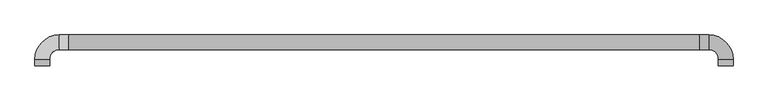
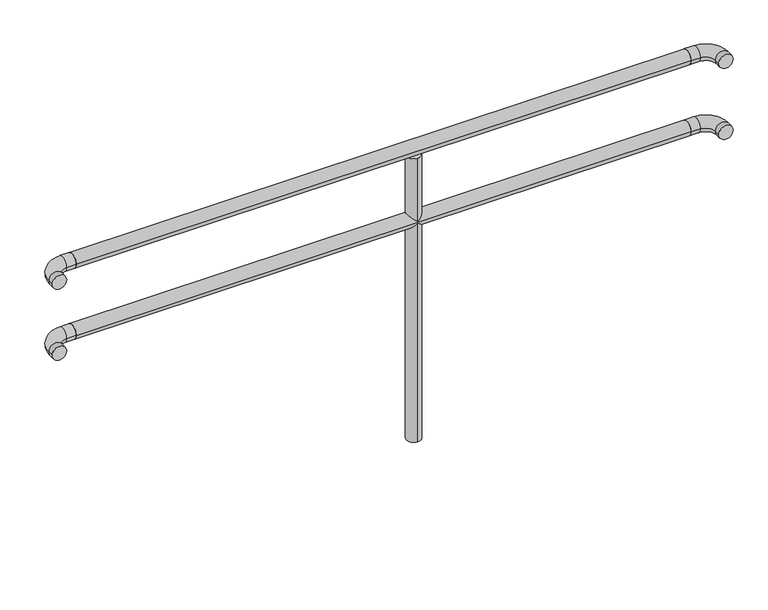
"""IFC4 building model written with IfcOpenShell, lengths in millimetres: railing geometry."""

from ifc_helpers import new_model, si_unit, point, frame, frame_2d, origin, origin_with_axes, place, context, project, spatial, circle_curve, ellipse_curve, trimmed, segment, composite_curve, outline, extrude, source, transform, mapped, element, save
from ifc_brep_helpers import plane_surface, cylinder_surface, revolved_surface, advanced_brep


def railing_ab6729c0(model_context):
    return source(origin(), model_context, "Body", "SolidModel", [
        extrude(outline(composite_curve([segment(trimmed(circle_curve(frame_2d((31458.1400611, 899.0)), 21.0), [point((31479.1400611, 899.0))], [point((31437.1400611, 899.0))], False, "CARTESIAN"), True, "CONTINUOUS"), segment(trimmed(circle_curve(frame_2d((31458.1400611, 899.0)), 21.0), [point((31437.1400611, 899.0))], [point((31479.1400611, 899.0))], False, "CARTESIAN"), True, "CONTINUOUS")], self_intersect=False)), frame((9766.6129185, 0.0, 0.0), z_axis=(1.0, 0.0, 0.0), x_axis=(0.0, 1.0, 0.0)), (0.0, 0.0, 1.0), 1800.0),
        extrude(outline(composite_curve([segment(trimmed(circle_curve(frame_2d((31458.1400611, 679.0)), 21.0), [point((31479.1400611, 679.0))], [point((31437.1400611, 679.0))], False, "CARTESIAN"), True, "CONTINUOUS"), segment(trimmed(circle_curve(frame_2d((31458.1400611, 679.0)), 21.0), [point((31437.1400611, 679.0))], [point((31479.1400611, 679.0))], False, "CARTESIAN"), True, "CONTINUOUS")], self_intersect=False)), frame((9766.6129185, 0.0, 0.0), z_axis=(1.0, 0.0, 0.0), x_axis=(0.0, 1.0, 0.0)), (0.0, 0.0, 1.0), 1800.0),
        extrude(outline(composite_curve([segment(trimmed(circle_curve(frame_2d((10766.6129185, 31458.1400611)), 21.0), [point((10766.6129185, 31479.1400611))], [point((10766.6129185, 31437.1400611))], False, "CARTESIAN"), True, "CONTINUOUS"), segment(trimmed(circle_curve(frame_2d((10766.6129185, 31458.1400611)), 21.0), [point((10766.6129185, 31437.1400611))], [point((10766.6129185, 31479.1400611))], False, "CARTESIAN"), True, "CONTINUOUS")], self_intersect=False)), origin_with_axes(), (0.0, 0.0, 1.0), 878.0),
        advanced_brep(
        [(11566.6129185, 31437.1900611, 679.1), (11566.6129185, 31479.1900611, 679.1), (11594.1129185, 31437.1900611, 679.1), (11594.1129185, 31479.1900611, 679.1), (11663.6129185, 31409.6900611, 679.1), (11621.6129185, 31409.6900611, 679.1), (11621.6129185, 31391.1900611, 679.1), (11663.6129185, 31391.1900611, 679.1)],
        [
            (0, 1, circle_curve(frame((11566.6129185, 31458.1900611, 679.1), z_axis=(-1.0, 0.0, 0.0), x_axis=(0.0, 1.0, 0.0)), 21.0)),
            (1, 0, circle_curve(frame((11566.6129185, 31458.1900611, 679.1), z_axis=(-1.0, 0.0, 0.0), x_axis=(0.0, 1.0, 0.0)), 21.0)),
            (0, 2),
            (2, 3, circle_curve(frame((11594.1129185, 31458.1900611, 679.1), z_axis=(-1.0, 0.0, 0.0), x_axis=(0.0, 1.0, 0.0)), 21.0)),
            (3, 1),
            (3, 2, circle_curve(frame((11594.1129185, 31458.1900611, 679.1), z_axis=(-1.0, 0.0, 0.0), x_axis=(0.0, 1.0, 0.0)), 21.0)),
            (4, 3, circle_curve(frame((11594.1129185, 31409.6900611, 679.1), z_axis=(0.0, 0.0, 1.0), x_axis=(0.0, 1.0, 0.0)), 69.5)),
            (2, 5, circle_curve(frame((11594.1129185, 31409.6900611, 679.1), z_axis=(0.0, 0.0, -1.0), x_axis=(0.0, 1.0, 0.0)), 27.5)),
            (5, 4, circle_curve(frame((11642.6129185, 31409.6900611, 679.1), z_axis=(0.0, 1.0, 0.0), x_axis=(1.0, 0.0, 0.0)), 21.0)),
            (4, 5, circle_curve(frame((11642.6129185, 31409.6900611, 679.1), z_axis=(0.0, 1.0, 0.0), x_axis=(1.0, 0.0, 0.0)), 21.0)),
            (6, 7, circle_curve(frame((11642.6129185, 31391.1900611, 679.1), z_axis=(0.0, -1.0, 0.0), x_axis=(1.0, 0.0, 0.0)), 21.0)),
            (7, 6, circle_curve(frame((11642.6129185, 31391.1900611, 679.1), z_axis=(0.0, -1.0, 0.0), x_axis=(1.0, 0.0, 0.0)), 21.0)),
            (5, 6),
            (7, 4),
        ],
        [
            plane_surface(frame((11566.6129185, 31458.1900611, 679.1), z_axis=(-1.0, 0.0, 0.0), x_axis=(0.0, 0.0, 1.0))),
            cylinder_surface(frame((11566.6129185, 31458.1900611, 679.1), z_axis=(-1.0, 0.0, 0.0), x_axis=(0.0, 1.0, 0.0)), 21.0),
            revolved_surface(trimmed(ellipse_curve(frame((11594.1129185, 31458.1900611, 679.1), z_axis=(-1.0, 0.0, 0.0), x_axis=(0.0, 1.0, 0.0)), 21.0, 21.0), [point((11594.1129185, 31437.1900611, 679.1))], [point((11594.1129185, 31479.1900611, 679.1))], True, "CARTESIAN"), (11594.1129185, 31409.6900611, 679.1), (0.0, 0.0, -1.0)),
            revolved_surface(trimmed(ellipse_curve(frame((11594.1129185, 31458.1900611, 679.1), z_axis=(-1.0, 0.0, 0.0), x_axis=(0.0, 1.0, 0.0)), 21.0, 21.0), [point((11594.1129185, 31479.1900611, 679.1))], [point((11594.1129185, 31437.1900611, 679.1))], True, "CARTESIAN"), (11594.1129185, 31409.6900611, 679.1), (0.0, 0.0, -1.0)),
            plane_surface(frame((11642.6129185, 31391.1900611, 679.1), z_axis=(0.0, -1.0, 0.0), x_axis=(0.0, 0.0, 1.0))),
            cylinder_surface(frame((11642.6129185, 31409.6900611, 679.1), z_axis=(0.0, 1.0, 0.0), x_axis=(1.0, 0.0, 0.0)), 21.0),
        ],
        [
            (0, [[1, 2]]),
            (1, [[-1, 3, 4, 5]]),
            (1, [[-2, -5, 6, -3]]),
            (2, [[7, -4, 8, 9]]),
            (3, [[-8, -6, -7, 10]]),
            (4, [[11, 12]]),
            (5, [[-9, 13, -12, 14]]),
            (5, [[-10, -14, -11, -13]]),
        ],
    ),
        advanced_brep(
        [(11566.6129185, 31437.1900611, 899.1), (11566.6129185, 31479.1900611, 899.1), (11594.1129185, 31437.1900611, 899.1), (11594.1129185, 31479.1900611, 899.1), (11663.6129185, 31409.6900611, 899.1), (11621.6129185, 31409.6900611, 899.1), (11621.6129185, 31391.1900611, 899.1), (11663.6129185, 31391.1900611, 899.1)],
        [
            (0, 1, circle_curve(frame((11566.6129185, 31458.1900611, 899.1), z_axis=(-1.0, 0.0, 0.0), x_axis=(0.0, 1.0, 0.0)), 21.0)),
            (1, 0, circle_curve(frame((11566.6129185, 31458.1900611, 899.1), z_axis=(-1.0, 0.0, 0.0), x_axis=(0.0, 1.0, 0.0)), 21.0)),
            (0, 2),
            (2, 3, circle_curve(frame((11594.1129185, 31458.1900611, 899.1), z_axis=(-1.0, 0.0, 0.0), x_axis=(0.0, 1.0, 0.0)), 21.0)),
            (3, 1),
            (3, 2, circle_curve(frame((11594.1129185, 31458.1900611, 899.1), z_axis=(-1.0, 0.0, 0.0), x_axis=(0.0, 1.0, 0.0)), 21.0)),
            (4, 3, circle_curve(frame((11594.1129185, 31409.6900611, 899.1), z_axis=(0.0, 0.0, 1.0), x_axis=(0.0, 1.0, 0.0)), 69.5)),
            (2, 5, circle_curve(frame((11594.1129185, 31409.6900611, 899.1), z_axis=(0.0, 0.0, -1.0), x_axis=(0.0, 1.0, 0.0)), 27.5)),
            (5, 4, circle_curve(frame((11642.6129185, 31409.6900611, 899.1), z_axis=(0.0, 1.0, 0.0), x_axis=(1.0, 0.0, 0.0)), 21.0)),
            (4, 5, circle_curve(frame((11642.6129185, 31409.6900611, 899.1), z_axis=(0.0, 1.0, 0.0), x_axis=(1.0, 0.0, 0.0)), 21.0)),
            (6, 7, circle_curve(frame((11642.6129185, 31391.1900611, 899.1), z_axis=(0.0, -1.0, 0.0), x_axis=(1.0, 0.0, 0.0)), 21.0)),
            (7, 6, circle_curve(frame((11642.6129185, 31391.1900611, 899.1), z_axis=(0.0, -1.0, 0.0), x_axis=(1.0, 0.0, 0.0)), 21.0)),
            (5, 6),
            (7, 4),
        ],
        [
            plane_surface(frame((11566.6129185, 31458.1900611, 899.1), z_axis=(-1.0, 0.0, 0.0), x_axis=(0.0, 0.0, 1.0))),
            cylinder_surface(frame((11566.6129185, 31458.1900611, 899.1), z_axis=(-1.0, 0.0, 0.0), x_axis=(0.0, 1.0, 0.0)), 21.0),
            revolved_surface(trimmed(ellipse_curve(frame((11594.1129185, 31458.1900611, 899.1), z_axis=(-1.0, 0.0, 0.0), x_axis=(0.0, 1.0, 0.0)), 21.0, 21.0), [point((11594.1129185, 31437.1900611, 899.1))], [point((11594.1129185, 31479.1900611, 899.1))], True, "CARTESIAN"), (11594.1129185, 31409.6900611, 899.1), (0.0, 0.0, -1.0)),
            revolved_surface(trimmed(ellipse_curve(frame((11594.1129185, 31458.1900611, 899.1), z_axis=(-1.0, 0.0, 0.0), x_axis=(0.0, 1.0, 0.0)), 21.0, 21.0), [point((11594.1129185, 31479.1900611, 899.1))], [point((11594.1129185, 31437.1900611, 899.1))], True, "CARTESIAN"), (11594.1129185, 31409.6900611, 899.1), (0.0, 0.0, -1.0)),
            plane_surface(frame((11642.6129185, 31391.1900611, 899.1), z_axis=(0.0, -1.0, 0.0), x_axis=(0.0, 0.0, 1.0))),
            cylinder_surface(frame((11642.6129185, 31409.6900611, 899.1), z_axis=(0.0, 1.0, 0.0), x_axis=(1.0, 0.0, 0.0)), 21.0),
        ],
        [
            (0, [[1, 2]]),
            (1, [[-1, 3, 4, 5]]),
            (1, [[-2, -5, 6, -3]]),
            (2, [[7, -4, 8, 9]]),
            (3, [[-8, -6, -7, 10]]),
            (4, [[11, 12]]),
            (5, [[-9, 13, -12, 14]]),
            (5, [[-10, -14, -11, -13]]),
        ],
    ),
        advanced_brep(
        [(9766.6129185, 31479.1900611, 679.1), (9766.6129185, 31437.1900611, 679.1), (9739.1129185, 31437.1900611, 679.1), (9739.1129185, 31479.1900611, 679.1), (9669.6129185, 31409.6900611, 679.1), (9711.6129185, 31409.6900611, 679.1), (9711.6129185, 31391.1900611, 679.1), (9669.6129185, 31391.1900611, 679.1)],
        [
            (0, 1, circle_curve(frame((9766.6129185, 31458.1900611, 679.1), z_axis=(1.0, 0.0, 0.0), x_axis=(0.0, -1.0, 0.0)), 21.0)),
            (1, 0, circle_curve(frame((9766.6129185, 31458.1900611, 679.1), z_axis=(1.0, 0.0, 0.0), x_axis=(0.0, -1.0, 0.0)), 21.0)),
            (1, 2),
            (2, 3, circle_curve(frame((9739.1129185, 31458.1900611, 679.1), z_axis=(1.0, 0.0, 0.0), x_axis=(0.0, -1.0, 0.0)), 21.0)),
            (3, 0),
            (3, 2, circle_curve(frame((9739.1129185, 31458.1900611, 679.1), z_axis=(1.0, 0.0, 0.0), x_axis=(0.0, -1.0, 0.0)), 21.0)),
            (4, 3, circle_curve(frame((9739.1129185, 31409.6900611, 679.1), z_axis=(0.0, 0.0, -1.0), x_axis=(0.0, 1.0, 0.0)), 69.5)),
            (2, 5, circle_curve(frame((9739.1129185, 31409.6900611, 679.1), z_axis=(0.0, 0.0, 1.0), x_axis=(0.0, 1.0, 0.0)), 27.5)),
            (5, 4, circle_curve(frame((9690.6129185, 31409.6900611, 679.1), z_axis=(0.0, 1.0, 0.0), x_axis=(1.0, 0.0, 0.0)), 21.0)),
            (4, 5, circle_curve(frame((9690.6129185, 31409.6900611, 679.1), z_axis=(0.0, 1.0, 0.0), x_axis=(1.0, 0.0, 0.0)), 21.0)),
            (5, 6),
            (6, 7, circle_curve(frame((9690.6129185, 31391.1900611, 679.1), z_axis=(0.0, 1.0, 0.0), x_axis=(1.0, 0.0, 0.0)), 21.0)),
            (7, 4),
            (7, 6, circle_curve(frame((9690.6129185, 31391.1900611, 679.1), z_axis=(0.0, 1.0, 0.0), x_axis=(1.0, 0.0, 0.0)), 21.0)),
        ],
        [
            plane_surface(frame((9766.6129185, 31458.1900611, 679.1), z_axis=(1.0, 0.0, 0.0), x_axis=(0.0, 0.0, 1.0))),
            cylinder_surface(frame((9766.6129185, 31458.1900611, 679.1), z_axis=(1.0, 0.0, 0.0), x_axis=(0.0, -1.0, 0.0)), 21.0),
            revolved_surface(trimmed(ellipse_curve(frame((9739.1129185, 31458.1900611, 679.1), z_axis=(1.0, 0.0, 0.0), x_axis=(0.0, -1.0, 0.0)), 21.0, 21.0), [point((9739.1129185, 31437.1900611, 679.1))], [point((9739.1129185, 31479.1900611, 679.1))], True, "CARTESIAN"), (9739.1129185, 31409.6900611, 679.1), (0.0, 0.0, 1.0)),
            revolved_surface(trimmed(ellipse_curve(frame((9739.1129185, 31458.1900611, 679.1), z_axis=(1.0, 0.0, 0.0), x_axis=(0.0, -1.0, 0.0)), 21.0, 21.0), [point((9739.1129185, 31479.1900611, 679.1))], [point((9739.1129185, 31437.1900611, 679.1))], True, "CARTESIAN"), (9739.1129185, 31409.6900611, 679.1), (0.0, 0.0, 1.0)),
            cylinder_surface(frame((9690.6129185, 31409.6900611, 679.1), z_axis=(0.0, 1.0, 0.0), x_axis=(1.0, 0.0, 0.0)), 21.0),
            plane_surface(frame((9690.6129185, 31391.1900611, 679.1), z_axis=(0.0, -1.0, 0.0), x_axis=(0.0, 0.0, 1.0))),
        ],
        [
            (0, [[1, 2]]),
            (1, [[-2, 3, 4, 5]]),
            (1, [[-1, -5, 6, -3]]),
            (2, [[7, -4, 8, 9]]),
            (3, [[-8, -6, -7, 10]]),
            (4, [[-9, 11, 12, 13]]),
            (4, [[-10, -13, 14, -11]]),
            (5, [[-12, -14]]),
        ],
    ),
        advanced_brep(
        [(9766.6129185, 31479.1900611, 899.1), (9766.6129185, 31437.1900611, 899.1), (9739.1129185, 31437.1900611, 899.1), (9739.1129185, 31479.1900611, 899.1), (9669.6129185, 31409.6900611, 899.1), (9711.6129185, 31409.6900611, 899.1), (9669.6129185, 31391.1900611, 899.1), (9711.6129185, 31391.1900611, 899.1)],
        [
            (0, 1, circle_curve(frame((9766.6129185, 31458.1900611, 899.1), z_axis=(1.0, 0.0, 0.0), x_axis=(0.0, -1.0, 0.0)), 21.0)),
            (1, 0, circle_curve(frame((9766.6129185, 31458.1900611, 899.1), z_axis=(1.0, 0.0, 0.0), x_axis=(0.0, -1.0, 0.0)), 21.0)),
            (1, 2),
            (2, 3, circle_curve(frame((9739.1129185, 31458.1900611, 899.1), z_axis=(1.0, 0.0, 0.0), x_axis=(0.0, -1.0, 0.0)), 21.0)),
            (3, 0),
            (3, 2, circle_curve(frame((9739.1129185, 31458.1900611, 899.1), z_axis=(1.0, 0.0, 0.0), x_axis=(0.0, -1.0, 0.0)), 21.0)),
            (4, 3, circle_curve(frame((9739.1129185, 31409.6900611, 899.1), z_axis=(0.0, 0.0, -1.0), x_axis=(0.0, 1.0, 0.0)), 69.5)),
            (2, 5, circle_curve(frame((9739.1129185, 31409.6900611, 899.1), z_axis=(0.0, 0.0, 1.0), x_axis=(0.0, 1.0, 0.0)), 27.5)),
            (5, 4, circle_curve(frame((9690.6129185, 31409.6900611, 899.1), z_axis=(0.0, 1.0, 0.0), x_axis=(1.0, 0.0, 0.0)), 21.0)),
            (4, 5, circle_curve(frame((9690.6129185, 31409.6900611, 899.1), z_axis=(0.0, 1.0, 0.0), x_axis=(1.0, 0.0, 0.0)), 21.0)),
            (6, 7, circle_curve(frame((9690.6129185, 31391.1900611, 899.1), z_axis=(0.0, -1.0, 0.0), x_axis=(1.0, 0.0, 0.0)), 21.0)),
            (7, 6, circle_curve(frame((9690.6129185, 31391.1900611, 899.1), z_axis=(0.0, -1.0, 0.0), x_axis=(1.0, 0.0, 0.0)), 21.0)),
            (5, 7),
            (6, 4),
        ],
        [
            plane_surface(frame((9766.6129185, 31458.1900611, 899.1), z_axis=(1.0, 0.0, 0.0), x_axis=(0.0, 0.0, 1.0))),
            cylinder_surface(frame((9766.6129185, 31458.1900611, 899.1), z_axis=(1.0, 0.0, 0.0), x_axis=(0.0, -1.0, 0.0)), 21.0),
            revolved_surface(trimmed(ellipse_curve(frame((9739.1129185, 31458.1900611, 899.1), z_axis=(1.0, 0.0, 0.0), x_axis=(0.0, -1.0, 0.0)), 21.0, 21.0), [point((9739.1129185, 31437.1900611, 899.1))], [point((9739.1129185, 31479.1900611, 899.1))], True, "CARTESIAN"), (9739.1129185, 31409.6900611, 899.1), (0.0, 0.0, 1.0)),
            revolved_surface(trimmed(ellipse_curve(frame((9739.1129185, 31458.1900611, 899.1), z_axis=(1.0, 0.0, 0.0), x_axis=(0.0, -1.0, 0.0)), 21.0, 21.0), [point((9739.1129185, 31479.1900611, 899.1))], [point((9739.1129185, 31437.1900611, 899.1))], True, "CARTESIAN"), (9739.1129185, 31409.6900611, 899.1), (0.0, 0.0, 1.0)),
            plane_surface(frame((9690.6129185, 31391.1900611, 899.1), z_axis=(0.0, -1.0, 0.0), x_axis=(0.0, 0.0, 1.0))),
            cylinder_surface(frame((9690.6129185, 31409.6900611, 899.1), z_axis=(0.0, 1.0, 0.0), x_axis=(1.0, 0.0, 0.0)), 21.0),
        ],
        [
            (0, [[1, 2]]),
            (1, [[-2, 3, 4, 5]]),
            (1, [[-1, -5, 6, -3]]),
            (2, [[7, -4, 8, 9]]),
            (3, [[-8, -6, -7, 10]]),
            (4, [[11, 12]]),
            (5, [[-9, 13, -11, 14]]),
            (5, [[-10, -14, -12, -13]]),
        ],
    ),
    ])


if __name__ == "__main__":
    model = new_model("IFC4")
    model_context = context("Model", 3, world=origin())
    ifc_project = project(units=[si_unit("LENGTHUNIT", "METRE", prefix="MILLI")], contexts=[model_context])
    site = spatial("IfcSite", under=ifc_project)
    building = spatial("IfcBuilding", under=site)
    placement = place(None, origin())
    railing_shape = railing_ab6729c0(model_context)
    element("IfcRailing", 1, at=placement, inside=building, context=model_context, shape_type="MappedRepresentation", body=[
        mapped(railing_shape, transform((0.0, 0.0, 0.0), x_axis=(1.0, 0.0, 0.0), y_axis=(0.0, 1.0, 0.0), z_axis=(0.0, 0.0, 1.0))),
    ])
    save(model, "model.ifc")

# Revit data of these elements
# Element 1 (IfcRailing)
#   Materials on its faces: "Ferro - Pintura Esmalte"
# Materials
#   "Ferro - Pintura Esmalte": class "Pintura", colour RGB 255 255 255, transparency 0, Cost = 0
